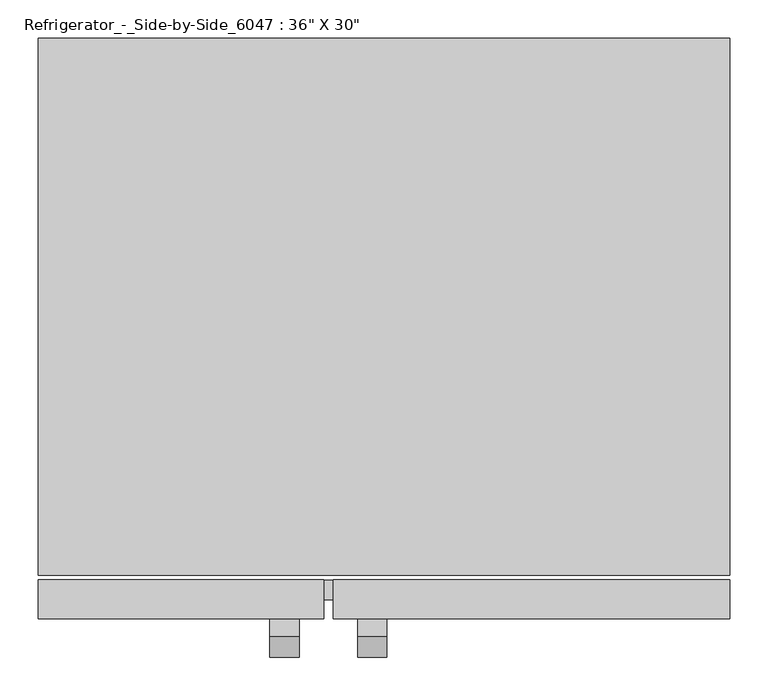
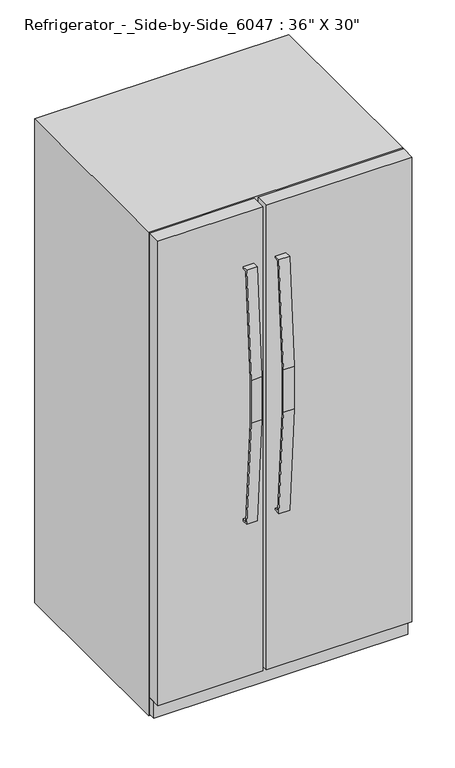
"""IFC4 building model written with IfcOpenShell, lengths in millimetres: proxy geometry."""

from ifc_helpers import new_model, si_unit, frame, origin, origin_with_axes, place, context, project, spatial, polyline, outline, extrude, source, transform, mapped, element, save


def proxy_32d0ea93(model_context):
    return source(origin(), model_context, "Body", "SweptSolid", [
        extrude(outline(polyline([(-440.1260285, 1226.3027548), (-440.1260285, 1065.4342469), (-412.6473987, 672.4715334), (-395.6760285, 672.4715334), (-395.6760285, 666.1370017), (-418.5699512, 666.1370017), (-446.4760285, 1065.2125), (-446.4760285, 1226.5245017), (-418.5699512, 1625.6), (-395.6760285, 1625.6), (-395.6760285, 1619.2654683), (-412.6473987, 1619.2654683), (-440.1260285, 1226.3027548)])), frame((-149.8915957, 0.0, 0.0), z_axis=(1.0, 0.0, 0.0), x_axis=(0.0, 1.0, 0.0)), (0.0, 0.0, 1.0), 38.4332978),
        extrude(outline(polyline([(-440.1260285, 1226.3027548), (-440.1260285, 1065.4342469), (-412.6473987, 672.4715334), (-395.6760285, 672.4715334), (-395.6760285, 666.1370017), (-418.5699512, 666.1370017), (-446.4760285, 1065.2125), (-446.4760285, 1226.5245017), (-418.5699512, 1625.6), (-395.6760285, 1625.6), (-395.6760285, 1619.2654683), (-412.6473987, 1619.2654683), (-440.1260285, 1226.3027548)])), frame((-34.5917022, 0.0, 0.0), z_axis=(1.0, 0.0, 0.0), x_axis=(0.0, 1.0, 0.0)), (0.0, 0.0, 1.0), 38.4332978),
        extrude(outline(polyline([(454.025, -344.8760285), (454.025, -370.2760285), (-454.025, -370.2760285), (-454.025, -344.8760285), (454.025, -344.8760285)])), frame((0.0, 0.0, 9.3816357), z_axis=(0.0, 0.0, 1.0), x_axis=(1.0, 0.0, 0.0)), (0.0, 0.0, 1.0), 63.5),
        extrude(outline(polyline([(454.025, 366.3239715), (454.025, -338.5260285), (-454.025, -338.5260285), (-454.025, 366.3239715), (454.025, 366.3239715)])), origin_with_axes(), (0.0, 0.0, 1.0), 1828.8),
        extrude(outline(polyline([(-79.375, -395.6760285), (-454.025, -395.6760285), (-454.025, -344.8760285), (-79.375, -344.8760285), (-79.375, -395.6760285)])), frame((0.0, 0.0, 72.8816357), z_axis=(0.0, 0.0, 1.0), x_axis=(1.0, 0.0, 0.0)), (0.0, 0.0, 1.0), 1755.9183643),
        extrude(outline(polyline([(454.025, -395.6760285), (-66.675, -395.6760285), (-66.675, -344.8760285), (454.025, -344.8760285), (454.025, -395.6760285)])), frame((0.0, 0.0, 72.8816357), z_axis=(0.0, 0.0, 1.0), x_axis=(1.0, 0.0, 0.0)), (0.0, 0.0, 1.0), 1755.9183643),
    ])


if __name__ == "__main__":
    model = new_model("IFC4")
    model_context = context("Model", 3, world=origin())
    ifc_project = project(units=[si_unit("LENGTHUNIT", "METRE", prefix="MILLI")], contexts=[model_context])
    site = spatial("IfcSite", under=ifc_project)
    building = spatial("IfcBuilding", under=site)
    placement = place(None, origin())
    proxy_shape = proxy_32d0ea93(model_context)
    element("IfcBuildingElementProxy", 1, Name="Refrigerator_-_Side-by-Side_6047 : 36\" X 30\"", ObjectType="Refrigerator_-_Side-by-Side_6047 : 36\" X 30\"", at=placement, inside=building, context=model_context, shape_type="MappedRepresentation", body=[
        mapped(proxy_shape, transform((0.0, 0.0, 0.0), x_axis=(1.0, 0.0, 0.0), y_axis=(0.0, 1.0, 0.0), z_axis=(0.0, 0.0, 1.0))),
    ])
    save(model, "model.ifc")

# Revit data of these elements
# Type "Refrigerator_-_Side-by-Side_6047 : 36\" X 30\""
#   Label = "REF."
#   Assembly Code = "E1090400"
#   Depth = 2' - 6"
#   Handle = 0' - 1 1/2"
#   Height = 6' - 0"
#   Rear Clearance = 0' - 2"
#   Top Door Height = 1' - 8"
#   Width = 2' - 11 3/4"
#   Base Material = none
#   Material = none
